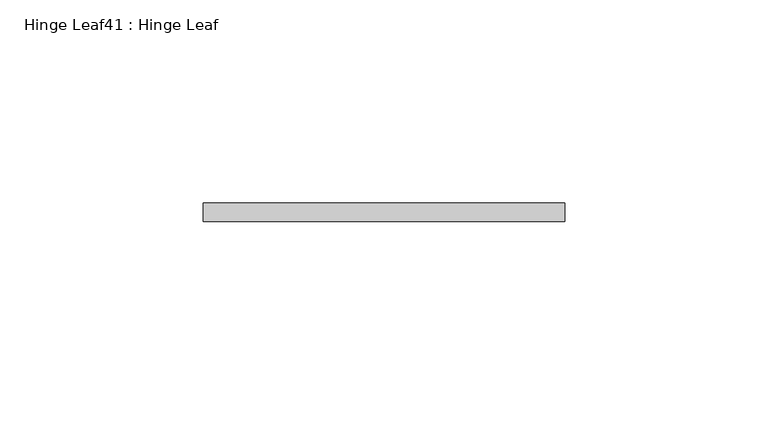
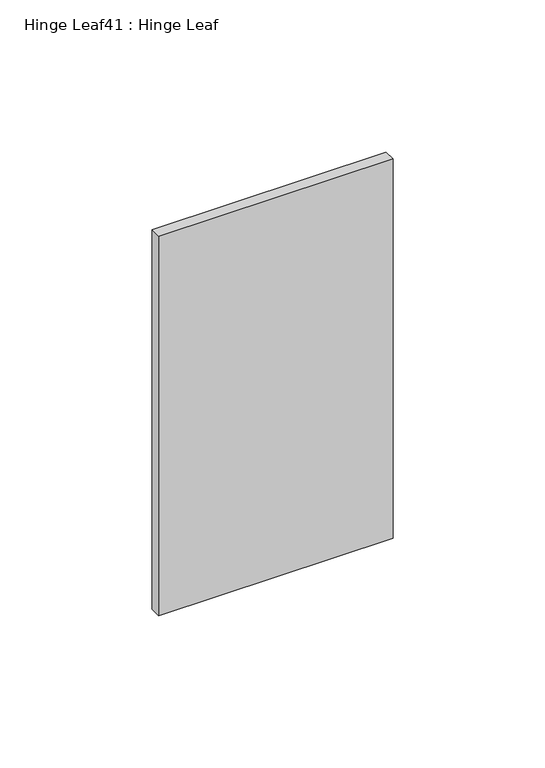
"""IFC4 building model written with IfcOpenShell, lengths in millimetres: proxy geometry, Hinge Leaf41 : Hinge Leaf."""

from ifc_helpers import new_model, si_unit, frame, origin, place, context, project, spatial, polyline, outline, extrude, source, transform, mapped, element, save


def hinge_leaf41_hinge_leaf_0c583ee0(model_context):
    return source(origin(), model_context, "Body", "SweptSolid", [
        extrude(outline(polyline([(587327.7934739, -534096.6663841), (587416.6934739, -534096.6663841), (587416.6934739, -534101.2383841), (587327.7934739, -534101.2383841), (587327.7934739, -534096.6663841)])), frame((0.0, 0.0, 1936.75), z_axis=(0.0, 0.0, 1.0), x_axis=(1.0, 0.0, 0.0)), (0.0, 0.0, 1.0), 152.4),
    ])


if __name__ == "__main__":
    model = new_model("IFC4")
    model_context = context("Model", 3, world=origin())
    ifc_project = project(units=[si_unit("LENGTHUNIT", "METRE", prefix="MILLI")], contexts=[model_context])
    site = spatial("IfcSite", under=ifc_project)
    building = spatial("IfcBuilding", under=site)
    placement = place(None, origin())
    hinge_leaf41_hinge_leaf_shape = hinge_leaf41_hinge_leaf_0c583ee0(model_context)
    element("IfcBuildingElementProxy", 1, Name="Hinge Leaf41 : Hinge Leaf", ObjectType="Hinge Leaf41 : Hinge Leaf", at=placement, inside=building, context=model_context, shape_type="MappedRepresentation", body=[
        mapped(hinge_leaf41_hinge_leaf_shape, transform((0.0, 0.0, 0.0), x_axis=(1.0, 0.0, 0.0), y_axis=(0.0, 1.0, 0.0), z_axis=(0.0, 0.0, 1.0))),
    ])
    save(model, "model.ifc")

# Revit data of these elements
# Element 1 (IfcBuildingElementProxy, "Hinge Leaf41 : Hinge Leaf")
#   Materials on its faces: "6\"X6\" WELD-ON STL BUTT HINGE"
# Materials
#   "6\"X6\" WELD-ON STL BUTT HINGE": class "Metal", colour RGB 189 187 185, transparency 0, Description = "Carbon steel", Cost = 0
